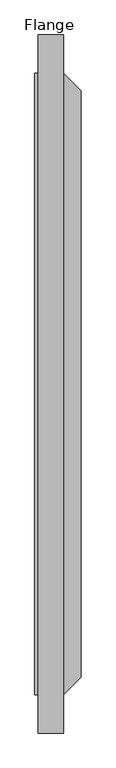
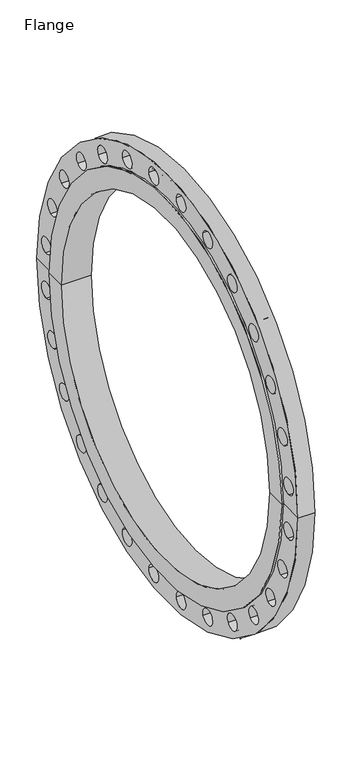
"""IFC4 building model written with IfcOpenShell, lengths in millimetres: proxy geometry, Flange : CASTED FLANGE PN16."""

from ifc_helpers import new_model, si_unit, frame, origin, place, context, project, spatial, polyline, circle_curve, source, transform, mapped, element, save
from ifc_brep_helpers import plane_surface, cylinder_surface, revolved_surface, advanced_brep


def flange_8ab1b455(model_context):
    return source(origin(), model_context, "Body", "AdvancedBrep", [
        advanced_brep(
        [(0.0, 450.0, 0.0), (0.0, 500.5, 0.0), (0.0, -500.5, 0.0), (0.0, -450.0, 0.0), (74.5, 450.0, 0.0), (74.5, -450.0, 0.0), (74.5, 472.5, 0.0), (74.5, -472.5, 0.0), (46.5, 500.5, 0.0), (46.5, -500.5, 0.0), (46.5, 562.5, 0.0), (46.5, -562.5, 0.0), (46.5, -79.1524503, -519.4036384), (46.5, -38.4102497, -523.994182), (46.5, 38.4102497, -523.994182), (46.5, 79.1524503, -519.4036384), (46.5, -192.7461158, -488.7680276), (46.5, -154.0468993, -502.3094692), (46.5, -523.994182, -38.4102497), (46.5, -519.4036384, -79.1524503), (46.5, -296.6746863, -433.623547), (46.5, -261.9589941, -455.4368622), (46.5, -385.7267491, -356.7353711), (46.5, -356.7353711, -385.7267491), (46.5, -455.4368622, -261.9589941), (46.5, -433.623547, -296.6746863), (46.5, -502.3094692, -154.0468993), (46.5, -488.7680276, -192.7461158), (46.5, 519.4036384, -79.1524503), (46.5, 523.994182, -38.4102497), (46.5, 488.7680276, -192.7461158), (46.5, 502.3094692, -154.0468993), (46.5, 433.623547, -296.6746863), (46.5, 455.4368622, -261.9589941), (46.5, 356.7353711, -385.7267491), (46.5, 385.7267491, -356.7353711), (46.5, 261.9589941, -455.4368622), (46.5, 296.6746863, -433.623547), (46.5, 154.0468993, -502.3094692), (46.5, 192.7461158, -488.7680276), (46.5, -433.623547, 296.6746863), (46.5, -455.4368622, 261.9589941), (46.5, -356.7353711, 385.7267491), (46.5, -385.7267491, 356.7353711), (46.5, -261.9589941, 455.4368622), (46.5, -296.6746863, 433.623547), (46.5, -154.0468993, 502.3094692), (46.5, -192.7461158, 488.7680276), (46.5, -38.4102497, 523.994182), (46.5, -79.1524503, 519.4036384), (46.5, 79.1524503, 519.4036384), (46.5, 38.4102497, 523.994182), (46.5, 192.7461158, 488.7680276), (46.5, 154.0468993, 502.3094692), (46.5, 296.6746863, 433.623547), (46.5, 261.9589941, 455.4368622), (46.5, 385.7267491, 356.7353711), (46.5, 356.7353711, 385.7267491), (46.5, 455.4368622, 261.9589941), (46.5, 433.623547, 296.6746863), (46.5, 502.3094692, 154.0468993), (46.5, 488.7680276, 192.7461158), (46.5, 523.994182, 38.4102497), (46.5, 519.4036384, 79.1524503), (46.5, -519.4036384, 79.1524503), (46.5, -523.994182, 38.4102497), (46.5, -488.7680276, 192.7461158), (46.5, -502.3094692, 154.0468993), (5.0, 562.5, 0.0), (5.0, -562.5, 0.0), (5.0, 500.5, 0.0), (5.0, -500.5, 0.0), (5.0, -38.4102497, -523.994182), (5.0, -79.1524503, -519.4036384), (5.0, 79.1524503, -519.4036384), (5.0, 38.4102497, -523.994182), (5.0, -154.0468993, -502.3094692), (5.0, -192.7461158, -488.7680276), (5.0, -519.4036384, -79.1524503), (5.0, -523.994182, -38.4102497), (5.0, -261.9589941, -455.4368622), (5.0, -296.6746863, -433.623547), (5.0, -356.7353711, -385.7267491), (5.0, -385.7267491, -356.7353711), (5.0, -433.623547, -296.6746863), (5.0, -455.4368622, -261.9589941), (5.0, -488.7680276, -192.7461158), (5.0, -502.3094692, -154.0468993), (5.0, 523.994182, -38.4102497), (5.0, 519.4036384, -79.1524503), (5.0, 502.3094692, -154.0468993), (5.0, 488.7680276, -192.7461158), (5.0, 455.4368622, -261.9589941), (5.0, 433.623547, -296.6746863), (5.0, 385.7267491, -356.7353711), (5.0, 356.7353711, -385.7267491), (5.0, 296.6746863, -433.623547), (5.0, 261.9589941, -455.4368622), (5.0, 192.7461158, -488.7680276), (5.0, 154.0468993, -502.3094692), (5.0, -455.4368622, 261.9589941), (5.0, -433.623547, 296.6746863), (5.0, -385.7267491, 356.7353711), (5.0, -356.7353711, 385.7267491), (5.0, -296.6746863, 433.623547), (5.0, -261.9589941, 455.4368622), (5.0, -192.7461158, 488.7680276), (5.0, -154.0468993, 502.3094692), (5.0, -79.1524503, 519.4036384), (5.0, -38.4102497, 523.994182), (5.0, 38.4102497, 523.994182), (5.0, 79.1524503, 519.4036384), (5.0, 154.0468993, 502.3094692), (5.0, 192.7461158, 488.7680276), (5.0, 261.9589941, 455.4368622), (5.0, 296.6746863, 433.623547), (5.0, 356.7353711, 385.7267491), (5.0, 385.7267491, 356.7353711), (5.0, 433.623547, 296.6746863), (5.0, 455.4368622, 261.9589941), (5.0, 488.7680276, 192.7461158), (5.0, 502.3094692, 154.0468993), (5.0, 519.4036384, 79.1524503), (5.0, 523.994182, 38.4102497), (5.0, -523.994182, 38.4102497), (5.0, -519.4036384, 79.1524503), (5.0, -502.3094692, 154.0468993), (5.0, -488.7680276, 192.7461158)],
        [
            (0, 1),
            (1, 2, circle_curve(frame((0.0, 0.0, 0.0), z_axis=(-1.0, 0.0, 0.0), x_axis=(0.0, 1.0, 0.0)), 500.5)),
            (2, 3),
            (3, 0, circle_curve(frame((0.0, 0.0, 0.0), z_axis=(1.0, 0.0, 0.0), x_axis=(0.0, 1.0, 0.0)), 450.0)),
            (0, 3, circle_curve(frame((0.0, 0.0, 0.0), z_axis=(1.0, 0.0, 0.0), x_axis=(0.0, 1.0, 0.0)), 450.0)),
            (2, 1, circle_curve(frame((0.0, 0.0, 0.0), z_axis=(-1.0, 0.0, 0.0), x_axis=(0.0, 1.0, 0.0)), 500.5)),
            (4, 0),
            (3, 5),
            (5, 4, circle_curve(frame((74.5, 0.0, 0.0), z_axis=(1.0, 0.0, 0.0), x_axis=(0.0, 1.0, 0.0)), 450.0)),
            (4, 5, circle_curve(frame((74.5, 0.0, 0.0), z_axis=(1.0, 0.0, 0.0), x_axis=(0.0, 1.0, 0.0)), 450.0)),
            (6, 4),
            (5, 7),
            (7, 6, circle_curve(frame((74.5, 0.0, 0.0), z_axis=(1.0, 0.0, 0.0), x_axis=(0.0, 1.0, 0.0)), 472.5)),
            (6, 7, circle_curve(frame((74.5, 0.0, 0.0), z_axis=(1.0, 0.0, 0.0), x_axis=(0.0, 1.0, 0.0)), 472.5)),
            (8, 6),
            (7, 9),
            (9, 8, circle_curve(frame((46.5, 0.0, 0.0), z_axis=(1.0, 0.0, 0.0), x_axis=(0.0, 1.0, 0.0)), 500.5)),
            (8, 9, circle_curve(frame((46.5, 0.0, 0.0), z_axis=(1.0, 0.0, 0.0), x_axis=(0.0, 1.0, 0.0)), 500.5)),
            (10, 8),
            (9, 11),
            (11, 10, circle_curve(frame((46.5, 0.0, 0.0), z_axis=(1.0, 0.0, 0.0), x_axis=(0.0, 1.0, 0.0)), 562.5)),
            (12, 13, circle_curve(frame((46.5, -58.78135, -521.6989102), z_axis=(-1.0, 0.0, 0.0), x_axis=(0.0, 0.9937122098932447, -0.11196447610328873)), 20.5)),
            (13, 12, circle_curve(frame((46.5, -58.78135, -521.6989102), z_axis=(-1.0, 0.0, 0.0), x_axis=(0.0, 0.9937122098932447, -0.11196447610328873)), 20.5)),
            (14, 15, circle_curve(frame((46.5, 58.78135, -521.6989102), z_axis=(-1.0, 0.0, 0.0), x_axis=(0.0, 0.9937122098932414, 0.1119644761033196)), 20.5)),
            (15, 14, circle_curve(frame((46.5, 58.78135, -521.6989102), z_axis=(-1.0, 0.0, 0.0), x_axis=(0.0, 0.9937122098932414, 0.1119644761033196)), 20.5)),
            (16, 17, circle_curve(frame((46.5, -173.3965075, -495.5387484), z_axis=(-1.0, 0.0, 0.0), x_axis=(0.0, 0.9438833303083805, -0.3302790619551306)), 20.5)),
            (17, 16, circle_curve(frame((46.5, -173.3965075, -495.5387484), z_axis=(-1.0, 0.0, 0.0), x_axis=(0.0, 0.9438833303083805, -0.3302790619551306)), 20.5)),
            (18, 19, circle_curve(frame((46.5, -521.6989102, -58.78135), z_axis=(-1.0, 0.0, 0.0), x_axis=(0.0, 0.11196447610332827, -0.9937122098932404)), 20.5)),
            (19, 18, circle_curve(frame((46.5, -521.6989102, -58.78135), z_axis=(-1.0, 0.0, 0.0), x_axis=(0.0, 0.11196447610332827, -0.9937122098932404)), 20.5)),
            (20, 21, circle_curve(frame((46.5, -279.3168402, -444.5302046), z_axis=(-1.0, 0.0, 0.0), x_axis=(0.0, 0.8467241992282982, -0.5320320765153143)), 20.5)),
            (21, 20, circle_curve(frame((46.5, -279.3168402, -444.5302046), z_axis=(-1.0, 0.0, 0.0), x_axis=(0.0, 0.8467241992282982, -0.5320320765153143)), 20.5)),
            (22, 23, circle_curve(frame((46.5, -371.2310601, -371.2310601), z_axis=(-1.0, 0.0, 0.0), x_axis=(0.0, 0.7071067811865616, -0.7071067811865335)), 20.5)),
            (23, 22, circle_curve(frame((46.5, -371.2310601, -371.2310601), z_axis=(-1.0, 0.0, 0.0), x_axis=(0.0, 0.7071067811865616, -0.7071067811865335)), 20.5)),
            (24, 25, circle_curve(frame((46.5, -444.5302046, -279.3168402), z_axis=(-1.0, 0.0, 0.0), x_axis=(0.0, 0.5320320765153537, -0.8467241992282734)), 20.5)),
            (25, 24, circle_curve(frame((46.5, -444.5302046, -279.3168402), z_axis=(-1.0, 0.0, 0.0), x_axis=(0.0, 0.5320320765153537, -0.8467241992282734)), 20.5)),
            (26, 27, circle_curve(frame((46.5, -495.5387484, -173.3965075), z_axis=(-1.0, 0.0, 0.0), x_axis=(0.0, 0.3302790619551865, -0.9438833303083608)), 20.5)),
            (27, 26, circle_curve(frame((46.5, -495.5387484, -173.3965075), z_axis=(-1.0, 0.0, 0.0), x_axis=(0.0, 0.3302790619551865, -0.9438833303083608)), 20.5)),
            (28, 29, circle_curve(frame((46.5, 521.6989102, -58.78135), z_axis=(-1.0, 0.0, 0.0), x_axis=(0.0, 0.11196447610327175, 0.9937122098932467)), 20.5)),
            (29, 28, circle_curve(frame((46.5, 521.6989102, -58.78135), z_axis=(-1.0, 0.0, 0.0), x_axis=(0.0, 0.11196447610327175, 0.9937122098932467)), 20.5)),
            (30, 31, circle_curve(frame((46.5, 495.5387484, -173.3965075), z_axis=(-1.0, 0.0, 0.0), x_axis=(0.0, 0.33027906195513196, 0.9438833303083799)), 20.5)),
            (31, 30, circle_curve(frame((46.5, 495.5387484, -173.3965075), z_axis=(-1.0, 0.0, 0.0), x_axis=(0.0, 0.33027906195513196, 0.9438833303083799)), 20.5)),
            (32, 33, circle_curve(frame((46.5, 444.5302046, -279.3168402), z_axis=(-1.0, 0.0, 0.0), x_axis=(0.0, 0.5320320765153052, 0.8467241992283039)), 20.5)),
            (33, 32, circle_curve(frame((46.5, 444.5302046, -279.3168402), z_axis=(-1.0, 0.0, 0.0), x_axis=(0.0, 0.5320320765153052, 0.8467241992283039)), 20.5)),
            (34, 35, circle_curve(frame((46.5, 371.2310601, -371.2310601), z_axis=(-1.0, 0.0, 0.0), x_axis=(0.0, 0.7071067811865214, 0.7071067811865739)), 20.5)),
            (35, 34, circle_curve(frame((46.5, 371.2310601, -371.2310601), z_axis=(-1.0, 0.0, 0.0), x_axis=(0.0, 0.7071067811865214, 0.7071067811865739)), 20.5)),
            (36, 37, circle_curve(frame((46.5, 279.3168402, -444.5302046), z_axis=(-1.0, 0.0, 0.0), x_axis=(0.0, 0.8467241992282644, 0.5320320765153681)), 20.5)),
            (37, 36, circle_curve(frame((46.5, 279.3168402, -444.5302046), z_axis=(-1.0, 0.0, 0.0), x_axis=(0.0, 0.8467241992282644, 0.5320320765153681)), 20.5)),
            (38, 39, circle_curve(frame((46.5, 173.3965075, -495.5387484), z_axis=(-1.0, 0.0, 0.0), x_axis=(0.0, 0.9438833303083553, 0.3302790619552022)), 20.5)),
            (39, 38, circle_curve(frame((46.5, 173.3965075, -495.5387484), z_axis=(-1.0, 0.0, 0.0), x_axis=(0.0, 0.9438833303083553, 0.3302790619552022)), 20.5)),
            (10, 11, circle_curve(frame((46.5, 0.0, 0.0), z_axis=(1.0, 0.0, 0.0), x_axis=(0.0, 1.0, 0.0)), 562.5)),
            (40, 41, circle_curve(frame((46.5, -444.5302046, 279.3168402), z_axis=(-1.0, 0.0, 0.0), x_axis=(0.0, -0.5320320765153187, -0.8467241992282954)), 20.5)),
            (41, 40, circle_curve(frame((46.5, -444.5302046, 279.3168402), z_axis=(-1.0, 0.0, 0.0), x_axis=(0.0, -0.5320320765153187, -0.8467241992282954)), 20.5)),
            (42, 43, circle_curve(frame((46.5, -371.2310601, 371.2310601), z_axis=(-1.0, 0.0, 0.0), x_axis=(0.0, -0.7071067811865323, -0.7071067811865629)), 20.5)),
            (43, 42, circle_curve(frame((46.5, -371.2310601, 371.2310601), z_axis=(-1.0, 0.0, 0.0), x_axis=(0.0, -0.7071067811865323, -0.7071067811865629)), 20.5)),
            (44, 45, circle_curve(frame((46.5, -279.3168402, 444.5302046), z_axis=(-1.0, 0.0, 0.0), x_axis=(0.0, -0.8467241992282726, -0.5320320765153552)), 20.5)),
            (45, 44, circle_curve(frame((46.5, -279.3168402, 444.5302046), z_axis=(-1.0, 0.0, 0.0), x_axis=(0.0, -0.8467241992282726, -0.5320320765153552)), 20.5)),
            (46, 47, circle_curve(frame((46.5, -173.3965075, 495.5387484), z_axis=(-1.0, 0.0, 0.0), x_axis=(0.0, -0.9438833303083604, -0.3302790619551879)), 20.5)),
            (47, 46, circle_curve(frame((46.5, -173.3965075, 495.5387484), z_axis=(-1.0, 0.0, 0.0), x_axis=(0.0, -0.9438833303083604, -0.3302790619551879)), 20.5)),
            (48, 49, circle_curve(frame((46.5, -58.78135, 521.6989102), z_axis=(-1.0, 0.0, 0.0), x_axis=(0.0, -0.9937122098932402, -0.11196447610332975)), 20.5)),
            (49, 48, circle_curve(frame((46.5, -58.78135, 521.6989102), z_axis=(-1.0, 0.0, 0.0), x_axis=(0.0, -0.9937122098932402, -0.11196447610332975)), 20.5)),
            (50, 51, circle_curve(frame((46.5, 58.78135, 521.6989102), z_axis=(-1.0, 0.0, 0.0), x_axis=(0.0, -0.9937122098932452, 0.11196447610328553)), 20.5)),
            (51, 50, circle_curve(frame((46.5, 58.78135, 521.6989102), z_axis=(-1.0, 0.0, 0.0), x_axis=(0.0, -0.9937122098932452, 0.11196447610328553)), 20.5)),
            (52, 53, circle_curve(frame((46.5, 173.3965075, 495.5387484), z_axis=(-1.0, 0.0, 0.0), x_axis=(0.0, -0.9438833303083796, 0.3302790619551329)), 20.5)),
            (53, 52, circle_curve(frame((46.5, 173.3965075, 495.5387484), z_axis=(-1.0, 0.0, 0.0), x_axis=(0.0, -0.9438833303083796, 0.3302790619551329)), 20.5)),
            (54, 55, circle_curve(frame((46.5, 279.3168402, 444.5302046), z_axis=(-1.0, 0.0, 0.0), x_axis=(0.0, -0.8467241992283037, 0.5320320765153059)), 20.5)),
            (55, 54, circle_curve(frame((46.5, 279.3168402, 444.5302046), z_axis=(-1.0, 0.0, 0.0), x_axis=(0.0, -0.8467241992283037, 0.5320320765153059)), 20.5)),
            (56, 57, circle_curve(frame((46.5, 371.2310601, 371.2310601), z_axis=(-1.0, 0.0, 0.0), x_axis=(0.0, -0.7071067811865736, 0.7071067811865215)), 20.5)),
            (57, 56, circle_curve(frame((46.5, 371.2310601, 371.2310601), z_axis=(-1.0, 0.0, 0.0), x_axis=(0.0, -0.7071067811865736, 0.7071067811865215)), 20.5)),
            (58, 59, circle_curve(frame((46.5, 444.5302046, 279.3168402), z_axis=(-1.0, 0.0, 0.0), x_axis=(0.0, -0.532032076515368, 0.8467241992282643)), 20.5)),
            (59, 58, circle_curve(frame((46.5, 444.5302046, 279.3168402), z_axis=(-1.0, 0.0, 0.0), x_axis=(0.0, -0.532032076515368, 0.8467241992282643)), 20.5)),
            (60, 61, circle_curve(frame((46.5, 495.5387484, 173.3965075), z_axis=(-1.0, 0.0, 0.0), x_axis=(0.0, -0.3302790619552013, 0.9438833303083556)), 20.5)),
            (61, 60, circle_curve(frame((46.5, 495.5387484, 173.3965075), z_axis=(-1.0, 0.0, 0.0), x_axis=(0.0, -0.3302790619552013, 0.9438833303083556)), 20.5)),
            (62, 63, circle_curve(frame((46.5, 521.6989102, 58.78135), z_axis=(-1.0, 0.0, 0.0), x_axis=(0.0, -0.111964476103344, 0.9937122098932386)), 20.5)),
            (63, 62, circle_curve(frame((46.5, 521.6989102, 58.78135), z_axis=(-1.0, 0.0, 0.0), x_axis=(0.0, -0.111964476103344, 0.9937122098932386)), 20.5)),
            (64, 65, circle_curve(frame((46.5, -521.6989102, 58.78135), z_axis=(-1.0, 0.0, 0.0), x_axis=(0.0, -0.11196447610328686, -0.9937122098932449)), 20.5)),
            (65, 64, circle_curve(frame((46.5, -521.6989102, 58.78135), z_axis=(-1.0, 0.0, 0.0), x_axis=(0.0, -0.11196447610328686, -0.9937122098932449)), 20.5)),
            (66, 67, circle_curve(frame((46.5, -495.5387484, 173.3965075), z_axis=(-1.0, 0.0, 0.0), x_axis=(0.0, -0.3302790619551471, -0.9438833303083745)), 20.5)),
            (67, 66, circle_curve(frame((46.5, -495.5387484, 173.3965075), z_axis=(-1.0, 0.0, 0.0), x_axis=(0.0, -0.3302790619551471, -0.9438833303083745)), 20.5)),
            (68, 10),
            (11, 69),
            (69, 68, circle_curve(frame((5.0, 0.0, 0.0), z_axis=(1.0, 0.0, 0.0), x_axis=(0.0, 1.0, 0.0)), 562.5)),
            (68, 69, circle_curve(frame((5.0, 0.0, 0.0), z_axis=(1.0, 0.0, 0.0), x_axis=(0.0, 1.0, 0.0)), 562.5)),
            (70, 68),
            (69, 71),
            (71, 70, circle_curve(frame((5.0, 0.0, 0.0), z_axis=(1.0, 0.0, 0.0), x_axis=(0.0, 1.0, 0.0)), 500.5)),
            (72, 73, circle_curve(frame((5.0, -58.78135, -521.6989102), z_axis=(1.0, 0.0, 0.0), x_axis=(0.0, 0.9937122098932447, -0.11196447610328873)), 20.5)),
            (73, 72, circle_curve(frame((5.0, -58.78135, -521.6989102), z_axis=(1.0, 0.0, 0.0), x_axis=(0.0, 0.9937122098932447, -0.11196447610328873)), 20.5)),
            (74, 75, circle_curve(frame((5.0, 58.78135, -521.6989102), z_axis=(1.0, 0.0, 0.0), x_axis=(0.0, 0.9937122098932414, 0.1119644761033196)), 20.5)),
            (75, 74, circle_curve(frame((5.0, 58.78135, -521.6989102), z_axis=(1.0, 0.0, 0.0), x_axis=(0.0, 0.9937122098932414, 0.1119644761033196)), 20.5)),
            (76, 77, circle_curve(frame((5.0, -173.3965075, -495.5387484), z_axis=(1.0, 0.0, 0.0), x_axis=(0.0, 0.9438833303083805, -0.3302790619551306)), 20.5)),
            (77, 76, circle_curve(frame((5.0, -173.3965075, -495.5387484), z_axis=(1.0, 0.0, 0.0), x_axis=(0.0, 0.9438833303083805, -0.3302790619551306)), 20.5)),
            (78, 79, circle_curve(frame((5.0, -521.6989102, -58.78135), z_axis=(1.0, 0.0, 0.0), x_axis=(0.0, 0.11196447610332827, -0.9937122098932404)), 20.5)),
            (79, 78, circle_curve(frame((5.0, -521.6989102, -58.78135), z_axis=(1.0, 0.0, 0.0), x_axis=(0.0, 0.11196447610332827, -0.9937122098932404)), 20.5)),
            (80, 81, circle_curve(frame((5.0, -279.3168402, -444.5302046), z_axis=(1.0, 0.0, 0.0), x_axis=(0.0, 0.8467241992282982, -0.5320320765153143)), 20.5)),
            (81, 80, circle_curve(frame((5.0, -279.3168402, -444.5302046), z_axis=(1.0, 0.0, 0.0), x_axis=(0.0, 0.8467241992282982, -0.5320320765153143)), 20.5)),
            (82, 83, circle_curve(frame((5.0, -371.2310601, -371.2310601), z_axis=(1.0, 0.0, 0.0), x_axis=(0.0, 0.7071067811865616, -0.7071067811865335)), 20.5)),
            (83, 82, circle_curve(frame((5.0, -371.2310601, -371.2310601), z_axis=(1.0, 0.0, 0.0), x_axis=(0.0, 0.7071067811865616, -0.7071067811865335)), 20.5)),
            (84, 85, circle_curve(frame((5.0, -444.5302046, -279.3168402), z_axis=(1.0, 0.0, 0.0), x_axis=(0.0, 0.5320320765153537, -0.8467241992282734)), 20.5)),
            (85, 84, circle_curve(frame((5.0, -444.5302046, -279.3168402), z_axis=(1.0, 0.0, 0.0), x_axis=(0.0, 0.5320320765153537, -0.8467241992282734)), 20.5)),
            (86, 87, circle_curve(frame((5.0, -495.5387484, -173.3965075), z_axis=(1.0, 0.0, 0.0), x_axis=(0.0, 0.3302790619551865, -0.9438833303083608)), 20.5)),
            (87, 86, circle_curve(frame((5.0, -495.5387484, -173.3965075), z_axis=(1.0, 0.0, 0.0), x_axis=(0.0, 0.3302790619551865, -0.9438833303083608)), 20.5)),
            (88, 89, circle_curve(frame((5.0, 521.6989102, -58.78135), z_axis=(1.0, 0.0, 0.0), x_axis=(0.0, 0.11196447610327175, 0.9937122098932467)), 20.5)),
            (89, 88, circle_curve(frame((5.0, 521.6989102, -58.78135), z_axis=(1.0, 0.0, 0.0), x_axis=(0.0, 0.11196447610327175, 0.9937122098932467)), 20.5)),
            (90, 91, circle_curve(frame((5.0, 495.5387484, -173.3965075), z_axis=(1.0, 0.0, 0.0), x_axis=(0.0, 0.33027906195513196, 0.9438833303083799)), 20.5)),
            (91, 90, circle_curve(frame((5.0, 495.5387484, -173.3965075), z_axis=(1.0, 0.0, 0.0), x_axis=(0.0, 0.33027906195513196, 0.9438833303083799)), 20.5)),
            (92, 93, circle_curve(frame((5.0, 444.5302046, -279.3168402), z_axis=(1.0, 0.0, 0.0), x_axis=(0.0, 0.5320320765153052, 0.8467241992283039)), 20.5)),
            (93, 92, circle_curve(frame((5.0, 444.5302046, -279.3168402), z_axis=(1.0, 0.0, 0.0), x_axis=(0.0, 0.5320320765153052, 0.8467241992283039)), 20.5)),
            (94, 95, circle_curve(frame((5.0, 371.2310601, -371.2310601), z_axis=(1.0, 0.0, 0.0), x_axis=(0.0, 0.7071067811865214, 0.7071067811865739)), 20.5)),
            (95, 94, circle_curve(frame((5.0, 371.2310601, -371.2310601), z_axis=(1.0, 0.0, 0.0), x_axis=(0.0, 0.7071067811865214, 0.7071067811865739)), 20.5)),
            (96, 97, circle_curve(frame((5.0, 279.3168402, -444.5302046), z_axis=(1.0, 0.0, 0.0), x_axis=(0.0, 0.8467241992282644, 0.5320320765153681)), 20.5)),
            (97, 96, circle_curve(frame((5.0, 279.3168402, -444.5302046), z_axis=(1.0, 0.0, 0.0), x_axis=(0.0, 0.8467241992282644, 0.5320320765153681)), 20.5)),
            (98, 99, circle_curve(frame((5.0, 173.3965075, -495.5387484), z_axis=(1.0, 0.0, 0.0), x_axis=(0.0, 0.9438833303083553, 0.3302790619552022)), 20.5)),
            (99, 98, circle_curve(frame((5.0, 173.3965075, -495.5387484), z_axis=(1.0, 0.0, 0.0), x_axis=(0.0, 0.9438833303083553, 0.3302790619552022)), 20.5)),
            (70, 71, circle_curve(frame((5.0, 0.0, 0.0), z_axis=(1.0, 0.0, 0.0), x_axis=(0.0, 1.0, 0.0)), 500.5)),
            (100, 101, circle_curve(frame((5.0, -444.5302046, 279.3168402), z_axis=(1.0, 0.0, 0.0), x_axis=(0.0, -0.5320320765153187, -0.8467241992282954)), 20.5)),
            (101, 100, circle_curve(frame((5.0, -444.5302046, 279.3168402), z_axis=(1.0, 0.0, 0.0), x_axis=(0.0, -0.5320320765153187, -0.8467241992282954)), 20.5)),
            (102, 103, circle_curve(frame((5.0, -371.2310601, 371.2310601), z_axis=(1.0, 0.0, 0.0), x_axis=(0.0, -0.7071067811865323, -0.7071067811865629)), 20.5)),
            (103, 102, circle_curve(frame((5.0, -371.2310601, 371.2310601), z_axis=(1.0, 0.0, 0.0), x_axis=(0.0, -0.7071067811865323, -0.7071067811865629)), 20.5)),
            (104, 105, circle_curve(frame((5.0, -279.3168402, 444.5302046), z_axis=(1.0, 0.0, 0.0), x_axis=(0.0, -0.8467241992282726, -0.5320320765153552)), 20.5)),
            (105, 104, circle_curve(frame((5.0, -279.3168402, 444.5302046), z_axis=(1.0, 0.0, 0.0), x_axis=(0.0, -0.8467241992282726, -0.5320320765153552)), 20.5)),
            (106, 107, circle_curve(frame((5.0, -173.3965075, 495.5387484), z_axis=(1.0, 0.0, 0.0), x_axis=(0.0, -0.9438833303083604, -0.3302790619551879)), 20.5)),
            (107, 106, circle_curve(frame((5.0, -173.3965075, 495.5387484), z_axis=(1.0, 0.0, 0.0), x_axis=(0.0, -0.9438833303083604, -0.3302790619551879)), 20.5)),
            (108, 109, circle_curve(frame((5.0, -58.78135, 521.6989102), z_axis=(1.0, 0.0, 0.0), x_axis=(0.0, -0.9937122098932402, -0.11196447610332975)), 20.5)),
            (109, 108, circle_curve(frame((5.0, -58.78135, 521.6989102), z_axis=(1.0, 0.0, 0.0), x_axis=(0.0, -0.9937122098932402, -0.11196447610332975)), 20.5)),
            (110, 111, circle_curve(frame((5.0, 58.78135, 521.6989102), z_axis=(1.0, 0.0, 0.0), x_axis=(0.0, -0.9937122098932452, 0.11196447610328553)), 20.5)),
            (111, 110, circle_curve(frame((5.0, 58.78135, 521.6989102), z_axis=(1.0, 0.0, 0.0), x_axis=(0.0, -0.9937122098932452, 0.11196447610328553)), 20.5)),
            (112, 113, circle_curve(frame((5.0, 173.3965075, 495.5387484), z_axis=(1.0, 0.0, 0.0), x_axis=(0.0, -0.9438833303083796, 0.3302790619551329)), 20.5)),
            (113, 112, circle_curve(frame((5.0, 173.3965075, 495.5387484), z_axis=(1.0, 0.0, 0.0), x_axis=(0.0, -0.9438833303083796, 0.3302790619551329)), 20.5)),
            (114, 115, circle_curve(frame((5.0, 279.3168402, 444.5302046), z_axis=(1.0, 0.0, 0.0), x_axis=(0.0, -0.8467241992283037, 0.5320320765153059)), 20.5)),
            (115, 114, circle_curve(frame((5.0, 279.3168402, 444.5302046), z_axis=(1.0, 0.0, 0.0), x_axis=(0.0, -0.8467241992283037, 0.5320320765153059)), 20.5)),
            (116, 117, circle_curve(frame((5.0, 371.2310601, 371.2310601), z_axis=(1.0, 0.0, 0.0), x_axis=(0.0, -0.7071067811865736, 0.7071067811865215)), 20.5)),
            (117, 116, circle_curve(frame((5.0, 371.2310601, 371.2310601), z_axis=(1.0, 0.0, 0.0), x_axis=(0.0, -0.7071067811865736, 0.7071067811865215)), 20.5)),
            (118, 119, circle_curve(frame((5.0, 444.5302046, 279.3168402), z_axis=(1.0, 0.0, 0.0), x_axis=(0.0, -0.532032076515368, 0.8467241992282643)), 20.5)),
            (119, 118, circle_curve(frame((5.0, 444.5302046, 279.3168402), z_axis=(1.0, 0.0, 0.0), x_axis=(0.0, -0.532032076515368, 0.8467241992282643)), 20.5)),
            (120, 121, circle_curve(frame((5.0, 495.5387484, 173.3965075), z_axis=(1.0, 0.0, 0.0), x_axis=(0.0, -0.3302790619552013, 0.9438833303083556)), 20.5)),
            (121, 120, circle_curve(frame((5.0, 495.5387484, 173.3965075), z_axis=(1.0, 0.0, 0.0), x_axis=(0.0, -0.3302790619552013, 0.9438833303083556)), 20.5)),
            (122, 123, circle_curve(frame((5.0, 521.6989102, 58.78135), z_axis=(1.0, 0.0, 0.0), x_axis=(0.0, -0.111964476103344, 0.9937122098932386)), 20.5)),
            (123, 122, circle_curve(frame((5.0, 521.6989102, 58.78135), z_axis=(1.0, 0.0, 0.0), x_axis=(0.0, -0.111964476103344, 0.9937122098932386)), 20.5)),
            (124, 125, circle_curve(frame((5.0, -521.6989102, 58.78135), z_axis=(1.0, 0.0, 0.0), x_axis=(0.0, -0.11196447610328686, -0.9937122098932449)), 20.5)),
            (125, 124, circle_curve(frame((5.0, -521.6989102, 58.78135), z_axis=(1.0, 0.0, 0.0), x_axis=(0.0, -0.11196447610328686, -0.9937122098932449)), 20.5)),
            (126, 127, circle_curve(frame((5.0, -495.5387484, 173.3965075), z_axis=(1.0, 0.0, 0.0), x_axis=(0.0, -0.3302790619551471, -0.9438833303083745)), 20.5)),
            (127, 126, circle_curve(frame((5.0, -495.5387484, 173.3965075), z_axis=(1.0, 0.0, 0.0), x_axis=(0.0, -0.3302790619551471, -0.9438833303083745)), 20.5)),
            (1, 70),
            (71, 2),
            (12, 73),
            (72, 13),
            (14, 75),
            (74, 15),
            (16, 77),
            (76, 17),
            (20, 81),
            (80, 21),
            (22, 83),
            (82, 23),
            (24, 85),
            (84, 25),
            (26, 87),
            (86, 27),
            (18, 79),
            (78, 19),
            (64, 125),
            (124, 65),
            (66, 127),
            (126, 67),
            (40, 101),
            (100, 41),
            (42, 103),
            (102, 43),
            (44, 105),
            (104, 45),
            (46, 107),
            (106, 47),
            (48, 109),
            (108, 49),
            (50, 111),
            (110, 51),
            (52, 113),
            (112, 53),
            (54, 115),
            (114, 55),
            (56, 117),
            (116, 57),
            (58, 119),
            (118, 59),
            (60, 121),
            (120, 61),
            (62, 123),
            (122, 63),
            (28, 89),
            (88, 29),
            (30, 91),
            (90, 31),
            (32, 93),
            (92, 33),
            (34, 95),
            (94, 35),
            (36, 97),
            (96, 37),
            (38, 99),
            (98, 39),
        ],
        [
            plane_surface(frame((0.0, 0.0, 0.0), z_axis=(-1.0, 0.0, 0.0), x_axis=(0.0, 1.0, 0.0))),
            revolved_surface(polyline([(0.0, 450.0, 0.0), (74.5, 450.0, 0.0)]), (-95.0, 0.0, 0.0), (-1.0, 0.0, 0.0)),
            plane_surface(frame((74.5, 0.0, 0.0), z_axis=(1.0, 0.0, 0.0), x_axis=(0.0, 1.0, 0.0))),
            revolved_surface(polyline([(74.5, 472.5, 0.0), (46.5, 500.5, 0.0)]), (-95.0, 0.0, 0.0), (-1.0, 0.0, 0.0)),
            plane_surface(frame((46.5, 0.0, 0.0), z_axis=(1.0, 0.0, 0.0), x_axis=(0.0, 1.0, 0.0))),
            cylinder_surface(frame((-95.0, 0.0, 0.0), z_axis=(-1.0, 0.0, 0.0), x_axis=(0.0, 1.0, 0.0)), 562.5),
            plane_surface(frame((5.0, 0.0, 0.0), z_axis=(-1.0, 0.0, 0.0), x_axis=(0.0, 1.0, 0.0))),
            cylinder_surface(frame((-95.0, 0.0, 0.0), z_axis=(-1.0, 0.0, 0.0), x_axis=(0.0, 1.0, 0.0)), 500.5),
            revolved_surface(polyline([(5.0, -38.41024969718849, -523.9941819601174), (46.5, -38.41024969718849, -523.9941819601174)]), (46.5, -58.78135, -521.6989102), (-1.0, 0.0, 0.0)),
            revolved_surface(polyline([(4.999999999999986, 79.15245030281145, -519.403638439882), (46.5, 79.15245030281145, -519.403638439882)]), (46.5, 58.78135, -521.6989102), (-1.0000000000000002, 0.0, 0.0)),
            revolved_surface(polyline([(4.999999999999986, -154.04689922867823, -502.30946917008015), (46.5, -154.04689922867823, -502.30946917008015)]), (46.5, -173.3965075, -495.5387484), (-1.0000000000000002, 0.0, 0.0)),
            revolved_surface(polyline([(5.0, -261.9589941158199, -455.43686216856395), (46.5, -261.9589941158199, -455.43686216856395)]), (46.5, -279.3168402, -444.5302046), (-1.0, 0.0, 0.0)),
            revolved_surface(polyline([(5.0, -356.73537108567547, -385.7267491143239), (46.5, -356.73537108567547, -385.7267491143239)]), (46.5, -371.2310601, -371.2310601), (-1.0, 0.0, 0.0)),
            revolved_surface(polyline([(5.0, -433.62354703143524, -296.6746862841796), (46.5, -433.62354703143524, -296.6746862841796)]), (46.5, -444.5302046, -279.3168402), (-1.0, 0.0, 0.0)),
            revolved_surface(polyline([(5.0, -488.76802762991866, -192.7461157713214), (46.5, -488.76802762991866, -192.7461157713214)]), (46.5, -495.5387484, -173.3965075), (-1.0, 0.0, 0.0)),
            revolved_surface(polyline([(4.999999999999986, -519.4036384398818, -79.15245030281143), (46.5, -519.4036384398818, -79.15245030281143)]), (46.5, -521.6989102, -58.78135), (-1.0000000000000002, 0.0, 0.0)),
            revolved_surface(polyline([(5.0, -523.9941819601174, 38.41024969718848), (46.5, -523.9941819601174, 38.41024969718848)]), (46.5, -521.6989102, 58.78135), (-1.0, 0.0, 0.0)),
            revolved_surface(polyline([(5.0, -502.3094691700805, 154.04689922867834), (46.5, -502.3094691700805, 154.04689922867834)]), (46.5, -495.5387484, 173.3965075), (-1.0, 0.0, 0.0)),
            revolved_surface(polyline([(5.0, -455.436862168564, 261.95899411581996), (46.5, -455.436862168564, 261.95899411581996)]), (46.5, -444.5302046, 279.3168402), (-1.0, 0.0, 0.0)),
            revolved_surface(polyline([(5.0, -385.72674911432387, 356.73537108567547), (46.5, -385.72674911432387, 356.73537108567547)]), (46.5, -371.2310601, 371.2310601), (-1.0, 0.0, 0.0)),
            revolved_surface(polyline([(4.999999999999986, -296.6746862841796, 433.62354703143524), (46.5, -296.6746862841796, 433.62354703143524)]), (46.5, -279.3168402, 444.5302046), (-1.0000000000000002, 0.0, 0.0)),
            revolved_surface(polyline([(4.999999999999986, -192.7461157713214, 488.7680276299186), (46.5, -192.7461157713214, 488.7680276299186)]), (46.5, -173.3965075, 495.5387484), (-1.0000000000000002, 0.0, 0.0)),
            revolved_surface(polyline([(5.0, -79.15245030281143, 519.4036384398818), (46.5, -79.15245030281143, 519.4036384398818)]), (46.5, -58.78135, 521.6989102), (-1.0, 0.0, 0.0)),
            revolved_surface(polyline([(5.0, 38.410249697188476, 523.9941819601173), (46.5, 38.410249697188476, 523.9941819601173)]), (46.5, 58.78135, 521.6989102), (-1.0, 0.0, 0.0)),
            revolved_surface(polyline([(4.999999999999986, 154.04689922867823, 502.3094691700802), (46.5, 154.04689922867823, 502.3094691700802)]), (46.5, 173.3965075, 495.5387484), (-1.0000000000000002, 0.0, 0.0)),
            revolved_surface(polyline([(4.999999999999986, 261.9589941158198, 455.4368621685638), (46.5, 261.9589941158198, 455.4368621685638)]), (46.5, 279.3168402, 444.5302046), (-1.0000000000000002, 0.0, 0.0)),
            revolved_surface(polyline([(5.0, 356.73537108567524, 385.7267491143237), (46.5, 356.73537108567524, 385.7267491143237)]), (46.5, 371.2310601, 371.2310601), (-1.0, 0.0, 0.0)),
            revolved_surface(polyline([(5.000000000000014, 433.62354703143495, 296.6746862841794), (46.5, 433.62354703143495, 296.6746862841794)]), (46.5, 444.5302046, 279.3168402), (-0.9999999999999998, 0.0, 0.0)),
            revolved_surface(polyline([(5.0, 488.7680276299183, 192.7461157713213), (46.5, 488.7680276299183, 192.7461157713213)]), (46.5, 495.5387484, 173.3965075), (-1.0, 0.0, 0.0)),
            revolved_surface(polyline([(4.999999999999986, 519.4036384398814, 79.15245030281139), (46.5, 519.4036384398814, 79.15245030281139)]), (46.5, 521.6989102, 58.78135), (-1.0000000000000002, 0.0, 0.0)),
            revolved_surface(polyline([(5.0, 523.9941819601171, -38.41024969718845), (46.5, 523.9941819601171, -38.41024969718845)]), (46.5, 521.6989102, -58.78135), (-1.0, 0.0, 0.0)),
            revolved_surface(polyline([(4.999999999999986, 502.3094691700802, -154.04689922867823), (46.5, 502.3094691700802, -154.04689922867823)]), (46.5, 495.5387484, -173.3965075), (-1.0000000000000002, 0.0, 0.0)),
            revolved_surface(polyline([(5.0, 455.4368621685637, -261.9589941158198), (46.5, 455.4368621685637, -261.9589941158198)]), (46.5, 444.5302046, -279.3168402), (-1.0, 0.0, 0.0)),
            revolved_surface(polyline([(4.999999999999986, 385.72674911432364, -356.73537108567524), (46.5, 385.72674911432364, -356.73537108567524)]), (46.5, 371.2310601, -371.2310601), (-1.0000000000000002, 0.0, 0.0)),
            revolved_surface(polyline([(5.0, 296.6746862841794, -433.62354703143495), (46.5, 296.6746862841794, -433.62354703143495)]), (46.5, 279.3168402, -444.5302046), (-1.0, 0.0, 0.0)),
            revolved_surface(polyline([(5.0, 192.74611577132129, -488.7680276299183), (46.5, 192.74611577132129, -488.7680276299183)]), (46.5, 173.3965075, -495.5387484), (-1.0, 0.0, 0.0)),
        ],
        [
            (0, [[1, 2, 3, 4]]),
            (0, [[-1, 5, -3, 6]]),
            (1, [[7, -4, 8, 9]]),
            (1, [[-7, 10, -8, -5]]),
            (2, [[11, -9, 12, 13]]),
            (2, [[-11, 14, -12, -10]]),
            (3, [[15, -13, 16, 17]]),
            (3, [[-15, 18, -16, -14]]),
            (4, [[19, -17, 20, 21], [22, 23], [24, 25], [26, 27], [28, 29], [30, 31], [32, 33], [34, 35], [36, 37], [38, 39], [40, 41], [42, 43], [44, 45], [46, 47], [48, 49]]),
            (4, [[-19, 50, -20, -18], [51, 52], [53, 54], [55, 56], [57, 58], [59, 60], [61, 62], [63, 64], [65, 66], [67, 68], [69, 70], [71, 72], [73, 74], [75, 76], [77, 78]]),
            (5, [[79, -21, 80, 81]]),
            (5, [[-79, 82, -80, -50]]),
            (6, [[83, -81, 84, 85], [86, 87], [88, 89], [90, 91], [92, 93], [94, 95], [96, 97], [98, 99], [100, 101], [102, 103], [104, 105], [106, 107], [108, 109], [110, 111], [112, 113]]),
            (6, [[-83, 114, -84, -82], [115, 116], [117, 118], [119, 120], [121, 122], [123, 124], [125, 126], [127, 128], [129, 130], [131, 132], [133, 134], [135, 136], [137, 138], [139, 140], [141, 142]]),
            (7, [[143, -85, 144, -2]]),
            (7, [[-143, -6, -144, -114]]),
            (8, [[145, -86, 146, -22]]),
            (8, [[-145, -23, -146, -87]]),
            (9, [[147, -88, 148, -24]]),
            (9, [[-147, -25, -148, -89]]),
            (10, [[149, -90, 150, -26]]),
            (10, [[-149, -27, -150, -91]]),
            (11, [[151, -94, 152, -30]]),
            (11, [[-151, -31, -152, -95]]),
            (12, [[153, -96, 154, -32]]),
            (12, [[-153, -33, -154, -97]]),
            (13, [[155, -98, 156, -34]]),
            (13, [[-155, -35, -156, -99]]),
            (14, [[157, -100, 158, -36]]),
            (14, [[-157, -37, -158, -101]]),
            (15, [[159, -92, 160, -28]]),
            (15, [[-159, -29, -160, -93]]),
            (16, [[161, -139, 162, -75]]),
            (16, [[-161, -76, -162, -140]]),
            (17, [[163, -141, 164, -77]]),
            (17, [[-163, -78, -164, -142]]),
            (18, [[165, -115, 166, -51]]),
            (18, [[-165, -52, -166, -116]]),
            (19, [[167, -117, 168, -53]]),
            (19, [[-167, -54, -168, -118]]),
            (20, [[169, -119, 170, -55]]),
            (20, [[-169, -56, -170, -120]]),
            (21, [[171, -121, 172, -57]]),
            (21, [[-171, -58, -172, -122]]),
            (22, [[173, -123, 174, -59]]),
            (22, [[-173, -60, -174, -124]]),
            (23, [[175, -125, 176, -61]]),
            (23, [[-175, -62, -176, -126]]),
            (24, [[177, -127, 178, -63]]),
            (24, [[-177, -64, -178, -128]]),
            (25, [[179, -129, 180, -65]]),
            (25, [[-179, -66, -180, -130]]),
            (26, [[181, -131, 182, -67]]),
            (26, [[-181, -68, -182, -132]]),
            (27, [[183, -133, 184, -69]]),
            (27, [[-183, -70, -184, -134]]),
            (28, [[185, -135, 186, -71]]),
            (28, [[-185, -72, -186, -136]]),
            (29, [[187, -137, 188, -73]]),
            (29, [[-187, -74, -188, -138]]),
            (30, [[189, -102, 190, -38]]),
            (30, [[-189, -39, -190, -103]]),
            (31, [[191, -104, 192, -40]]),
            (31, [[-191, -41, -192, -105]]),
            (32, [[193, -106, 194, -42]]),
            (32, [[-193, -43, -194, -107]]),
            (33, [[195, -108, 196, -44]]),
            (33, [[-195, -45, -196, -109]]),
            (34, [[197, -110, 198, -46]]),
            (34, [[-197, -47, -198, -111]]),
            (35, [[199, -112, 200, -48]]),
            (35, [[-199, -49, -200, -113]]),
        ],
    ),
    ])


if __name__ == "__main__":
    model = new_model("IFC4")
    model_context = context("Model", 3, world=origin())
    ifc_project = project(units=[si_unit("LENGTHUNIT", "METRE", prefix="MILLI")], contexts=[model_context])
    site = spatial("IfcSite", under=ifc_project)
    building = spatial("IfcBuilding", under=site)
    placement = place(None, origin())
    flange_shape = flange_8ab1b455(model_context)
    element("IfcBuildingElementProxy", 1, Name="Flange : CASTED FLANGE PN16", ObjectType="Flange : CASTED FLANGE PN16", at=placement, inside=building, context=model_context, shape_type="MappedRepresentation", body=[
        mapped(flange_shape, transform((0.0, 0.0, 0.0), x_axis=(1.0, 0.0, 0.0), y_axis=(0.0, 1.0, 0.0), z_axis=(0.0, 0.0, 1.0))),
    ])
    save(model, "model.ifc")

# Revit data of these elements
# Type "Flange : CASTED FLANGE PN16"
#   TABLE_DIMENSIONS = "DIMENSIONS FIXED FLANGE"
#   Short Description = ""
#   Description = "FIXED FLANGE"
#   K [instance default] = 110 mm
#   HOLE DIAMETER [instance default] = 19 mm
#   D4 [instance default] = 84 mm
#   DRILL DIAMETER [instance default] = 110 mm
#   DN [instance default] = 40 mm
#   D2 [instance default] = 70 mm
#   D [instance default] = 150 mm
#   f [instance default] = 3 mm
#   b [instance default] = 16 mm
#   ANGLE [instance default] = 45.00°
#   a [instance default] = 19 mm
#   PN = 16
#   BOLTS NUMBER [instance default] = 4
#   MATERIAL [instance default] = none
#   COATING [instance default] = none
#   Default Elevation = 0
# Element 1 (IfcBuildingElementProxy, "Flange : CASTED FLANGE PN16")
#   K = 1050 mm
#   HOLE DIAMETER = 41 mm
#   D4 = 1001 mm
#   DRILL DIAMETER = 1050 mm
#   DN = 900 mm
#   D2 = 945 mm
#   D = 1125 mm
#   f = 5 mm
#   b = 41.5 mm
#   a = 46.5 mm
#   BOLTS NUMBER = 28
#   COATING = Not informed
#   Materials on its faces: "Not informed"
# Materials
#   "Not informed": class "Paint/Coating", colour RGB 0 56 123, transparency 0, Description = "Not Informed", Cost = 0
